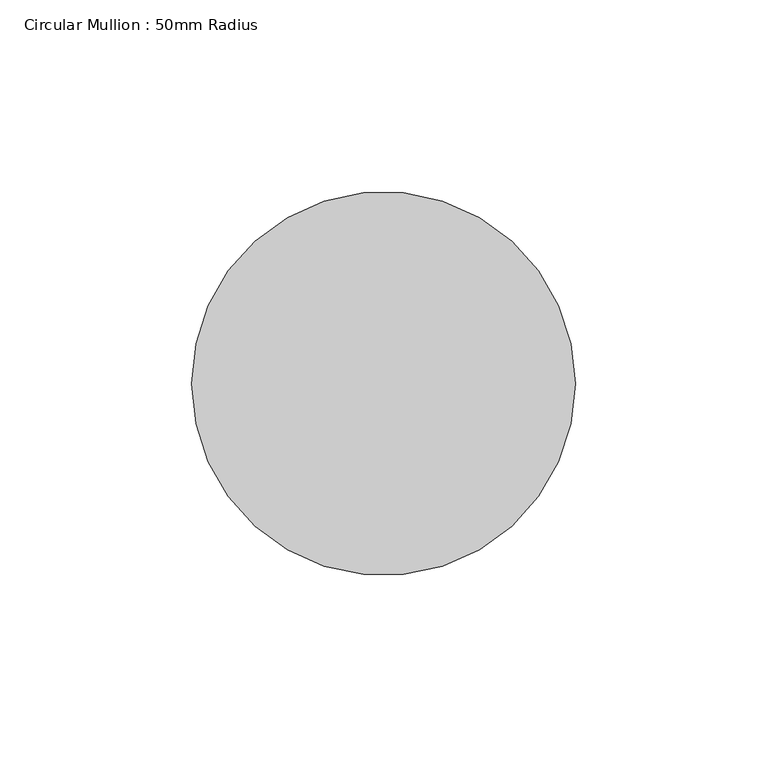
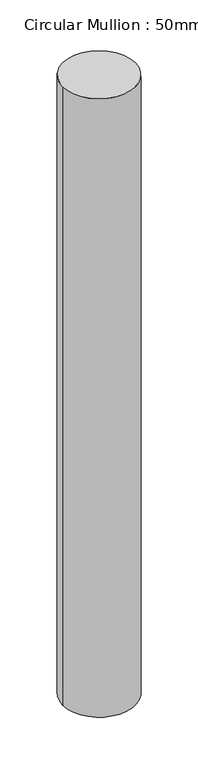
"""IFC4 building model written with IfcOpenShell, lengths in millimetres: member geometry, Circular Mullion : 50mm Radius."""

import ifcopenshell
import ifcopenshell.guid

model = None  # the IFC model being written
_history = None  # IfcOwnerHistory: only IFC2X3 demands one
_inside = {}  # id of a spatial element -> (the spatial element, [elements in it])
_under = {}  # id of a project, library or spatial element -> (it, [spatial elements below it])
_declared = {}  # id of a project -> (the project, [libraries it declares])
_typed = {}  # id of a type object -> (the type object, [elements of that type])
_made_of = {}  # id of a material, layer set ... -> (it, [elements and type objects made of it])


def new_model(schema):
    """Start an empty IFC model of exactly this schema.

    Asked for "IFC4X3", IfcOpenShell would pick the latest addendum, in which some entities
    have other attributes; the version numbers below select the first issue.
    IFC2X3 requires an IfcOwnerHistory on every rooted entity: one is made here for all.
    """
    global model, _history
    if schema == "IFC4X3":
        model = ifcopenshell.file(schema_version=(4, 3, 0, 0))
    else:
        model = ifcopenshell.file(schema=schema)
    _inside.clear()
    _under.clear()
    _declared.clear()
    _typed.clear()
    _made_of.clear()
    _history = None
    if model.schema == "IFC2X3":
        org = make("IfcOrganization", Name="unknown")
        user = make(
            "IfcPersonAndOrganization",
            ThePerson=make("IfcPerson", FamilyName="unknown"),
            TheOrganization=org,
        )
        app = make(
            "IfcApplication",
            ApplicationDeveloper=org,
            Version="unknown",
            ApplicationFullName="unknown",
            ApplicationIdentifier="unknown",
        )
        _history = make(
            "IfcOwnerHistory",
            OwningUser=user,
            OwningApplication=app,
            ChangeAction="ADDED",
            CreationDate=0,
        )
    return model


def make(cls, **values):
    """One entity of the class cls with the attributes given. An attribute that is None is left unset."""
    return model.create_entity(
        cls, **{name: value for name, value in values.items() if value is not None}
    )


def rooted(cls, **values):
    """An entity with a GlobalId (a new one), such as an element, a storey or a relation."""
    return make(cls, GlobalId=ifcopenshell.guid.new(), OwnerHistory=_history, **values)


def si_unit(unit_type, name, prefix=None):
    """IfcSIUnit, for example si_unit("LENGTHUNIT", "METRE", prefix="MILLI")."""
    return make("IfcSIUnit", UnitType=unit_type, Prefix=prefix, Name=name)


def assignment(units):
    """IfcUnitAssignment: the units of a project."""
    return None if units is None else make("IfcUnitAssignment", Units=units)


def point(xyz):
    """IfcCartesianPoint."""
    return None if xyz is None else make("IfcCartesianPoint", Coordinates=xyz)


def direction(xyz):
    """IfcDirection."""
    return None if xyz is None else make("IfcDirection", DirectionRatios=xyz)


def frame(location, z_axis=None, x_axis=None):
    """IfcAxis2Placement3D, a coordinate frame: its origin and axes. An axis left out is left unset."""
    return make(
        "IfcAxis2Placement3D",
        Location=point(location),
        Axis=direction(z_axis),
        RefDirection=direction(x_axis),
    )


def frame_2d(location, x_axis=None):
    """IfcAxis2Placement2D, a coordinate frame in the plane: its origin and x axis."""
    return make(
        "IfcAxis2Placement2D", Location=point(location), RefDirection=direction(x_axis)
    )


def origin():
    """The frame at (0, 0, 0) with its axes left unset."""
    return frame((0.0, 0.0, 0.0))


def origin_2d():
    """The frame at (0, 0) in the plane with its x axis left unset."""
    return frame_2d((0.0, 0.0))


def place(relative_to, where):
    """IfcLocalPlacement: puts the frame where relative to a parent placement (None: the world)."""
    return make(
        "IfcLocalPlacement", PlacementRelTo=relative_to, RelativePlacement=where
    )


def context(
    kind, dimensions, precision=None, world=None, true_north=None, identifier=None
):
    """IfcGeometricRepresentationContext, for example the 3D "Model" context."""
    return make(
        "IfcGeometricRepresentationContext",
        ContextIdentifier=identifier,
        ContextType=kind,
        CoordinateSpaceDimension=dimensions,
        Precision=precision,
        WorldCoordinateSystem=world,
        TrueNorth=true_north,
    )


def project(units=None, contexts=None):
    """IfcProject with its units and contexts."""
    return rooted(
        "IfcProject",
        Name="project",
        RepresentationContexts=contexts,
        UnitsInContext=assignment(units),
    )


def spatial(cls, under=None, at=None, **own):
    """A site, building, storey or space (cls), placed at a placement, below another one or the project."""
    s = rooted(cls, ObjectPlacement=at, **own)
    if under is not None:
        _under.setdefault(under.id(), (under, []))[1].append(s)
    return s


def circle_curve(where, radius):
    """IfcCircle in the frame where."""
    return make("IfcCircle", Position=where, Radius=radius)


def trimmed(basis, trim1, trim2, sense, master):
    """IfcTrimmedCurve: the piece of a basis curve between two trims."""
    return make(
        "IfcTrimmedCurve",
        BasisCurve=basis,
        Trim1=trim1,
        Trim2=trim2,
        SenseAgreement=sense,
        MasterRepresentation=master,
    )


def segment(curve, same_sense, transition):
    """IfcCompositeCurveSegment."""
    return make(
        "IfcCompositeCurveSegment",
        Transition=transition,
        SameSense=same_sense,
        ParentCurve=curve,
    )


def composite_curve(segments, self_intersect=None):
    """IfcCompositeCurve: segments joined end to end."""
    return make("IfcCompositeCurve", Segments=segments, SelfIntersect=self_intersect)


def outline(outer, holes=None, kind="AREA"):
    """IfcArbitraryClosedProfileDef: a profile drawn as a closed curve; with holes, ...WithVoids."""
    if holes is None:
        return make("IfcArbitraryClosedProfileDef", ProfileType=kind, OuterCurve=outer)
    return make(
        "IfcArbitraryProfileDefWithVoids",
        ProfileType=kind,
        OuterCurve=outer,
        InnerCurves=holes,
    )


def extrude(swept, where, along, depth):
    """IfcExtrudedAreaSolid: the profile swept, set in the frame where, extruded along a direction by depth."""
    return make(
        "IfcExtrudedAreaSolid",
        SweptArea=swept,
        Position=where,
        ExtrudedDirection=direction(along),
        Depth=depth,
    )


def shape(context_of_items, identifier, shape_type, items):
    """IfcShapeRepresentation: the items that make up one representation, for example the "Body"."""
    return make(
        "IfcShapeRepresentation",
        ContextOfItems=context_of_items,
        RepresentationIdentifier=identifier,
        RepresentationType=shape_type,
        Items=items,
    )


def source(mapping_origin, context_of_items, identifier, shape_type, items):
    """IfcRepresentationMap: a shape defined once, which mapped items show again and again."""
    return make(
        "IfcRepresentationMap",
        MappingOrigin=mapping_origin,
        MappedRepresentation=shape(context_of_items, identifier, shape_type, items),
    )


def transform(
    local_origin,
    x_axis=None,
    y_axis=None,
    z_axis=None,
    scale=None,
    scale2=None,
    scale3=None,
    uniform=True,
):
    """IfcCartesianTransformationOperator3D, or its non-uniform kind. x_axis, y_axis, z_axis: its Axis1, 2, 3."""
    if uniform:
        return make(
            "IfcCartesianTransformationOperator3D",
            Axis1=direction(x_axis),
            Axis2=direction(y_axis),
            LocalOrigin=point(local_origin),
            Scale=scale,
            Axis3=direction(z_axis),
        )
    return make(
        "IfcCartesianTransformationOperator3DnonUniform",
        Axis1=direction(x_axis),
        Axis2=direction(y_axis),
        LocalOrigin=point(local_origin),
        Scale=scale,
        Axis3=direction(z_axis),
        Scale2=scale2,
        Scale3=scale3,
    )


def mapped(mapping_source, mapping_target):
    """IfcMappedItem: shows the shape of a source again, moved by a transform."""
    return make(
        "IfcMappedItem", MappingSource=mapping_source, MappingTarget=mapping_target
    )


def made_of(thing, what):
    """Note that an element or type object is made of a material, layer set ...; save() writes the relation."""
    if what is not None:
        _made_of.setdefault(what.id(), (what, []))[1].append(thing)
    return thing


def element(
    cls,
    number,
    at=None,
    inside=None,
    cuts=None,
    type_object=None,
    material=None,
    context=None,
    identifier="Body",
    shape_type=None,
    held_by="IfcProductDefinitionShape",
    body=None,
    shapes=None,
    **own,
):
    """One element of the class cls, such as IfcWall. Its Tag is "e" and its number.

    at: its placement. inside: the storey or other place that contains it. cuts: it is an
    opening in that element (IfcRelVoidsElement). A single representation is given by context,
    identifier, shape_type and body (its items); several are given by shapes. held_by: the class
    of the entity that holds the representations. save() writes the other relations.
    """
    e = rooted(cls, Tag="e%d" % number, ObjectPlacement=at, **own)
    if body is not None:
        shapes = [shape(context, identifier, shape_type, body)]
    if shapes is not None:
        e.Representation = make(held_by, Representations=shapes)
    if inside is not None:
        _inside.setdefault(inside.id(), (inside, []))[1].append(e)
    if cuts is not None:
        rooted(
            "IfcRelVoidsElement", RelatingBuildingElement=cuts, RelatedOpeningElement=e
        )
    if type_object is not None:
        _typed.setdefault(type_object.id(), (type_object, []))[1].append(e)
    return made_of(e, material)


def aggregate(whole, parts):
    """IfcRelAggregates: a whole, such as a stair, and the parts it consists of."""
    return rooted("IfcRelAggregates", RelatingObject=whole, RelatedObjects=parts)


def save(model, path):
    """Write the relations noted so far, then the file.

    IfcRelAggregates (storeys below a building ...), IfcRelContainedInSpatialStructure (elements
    in a storey), IfcRelDefinesByType, IfcRelAssociatesMaterial and IfcRelDeclares: one each for
    every whole, place, type object, material and project.
    """
    for whole, parts in _under.values():
        aggregate(whole, parts)
    for where, things in _inside.values():
        rooted(
            "IfcRelContainedInSpatialStructure",
            RelatedElements=things,
            RelatingStructure=where,
        )
    for kind, things in _typed.values():
        rooted("IfcRelDefinesByType", RelatedObjects=things, RelatingType=kind)
    for what, things in _made_of.values():
        rooted("IfcRelAssociatesMaterial", RelatedObjects=things, RelatingMaterial=what)
    for by, libraries in _declared.values():
        rooted("IfcRelDeclares", RelatingContext=by, RelatedDefinitions=libraries)
    model.write(path)


def circular_mullion_50mm_radius_3c3aadbb(model_context):
    return source(origin(), model_context, "Body", "SweptSolid", [
        extrude(outline(composite_curve([segment(trimmed(circle_curve(origin_2d(), 50.0), [point((50.0, 0.0))], [point((-50.0, 0.0))], False, "CARTESIAN"), True, "CONTINUOUS"), segment(trimmed(circle_curve(origin_2d(), 50.0), [point((-50.0, 0.0))], [point((50.0, 0.0))], False, "CARTESIAN"), True, "CONTINUOUS")], self_intersect=False)), frame((0.0, 0.0, -899.9341667), z_axis=(0.0, 0.0, 1.0), x_axis=(1.0, 0.0, 0.0)), (0.0, 0.0, 1.0), 899.9341667),
    ])


if __name__ == "__main__":
    model = new_model("IFC4")
    model_context = context("Model", 3, world=origin())
    ifc_project = project(units=[si_unit("LENGTHUNIT", "METRE", prefix="MILLI")], contexts=[model_context])
    site = spatial("IfcSite", under=ifc_project)
    building = spatial("IfcBuilding", under=site)
    placement = place(None, origin())
    circular_mullion_50mm_radius_shape = circular_mullion_50mm_radius_3c3aadbb(model_context)
    element("IfcMember", 1, ObjectType="Circular Mullion : 50mm Radius", at=placement, inside=building, context=model_context, shape_type="MappedRepresentation", body=[
        mapped(circular_mullion_50mm_radius_shape, transform((0.0, 0.0, 0.0), x_axis=(1.0, 0.0, 0.0), y_axis=(0.0, 1.0, 0.0), z_axis=(0.0, 0.0, 1.0))),
    ])
    save(model, "model.ifc")

# Revit data of these elements
# Type "Circular Mullion : 50mm Radius"
#   built-in parameter 1007350 = 0.164042 (stored number, unit not read)
# Element 1 (IfcMember, "Circular Mullion : 50mm Radius")
#   Materials on its faces: "Aluminium"
# Materials
#   "Aluminium": class "Metal", colour RGB 247 247 247, transparency 0, Description = "Aluminium 6061", Cost = 0
